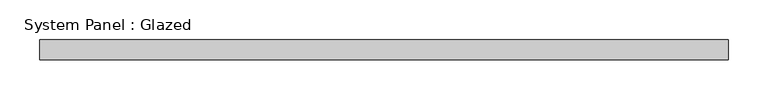
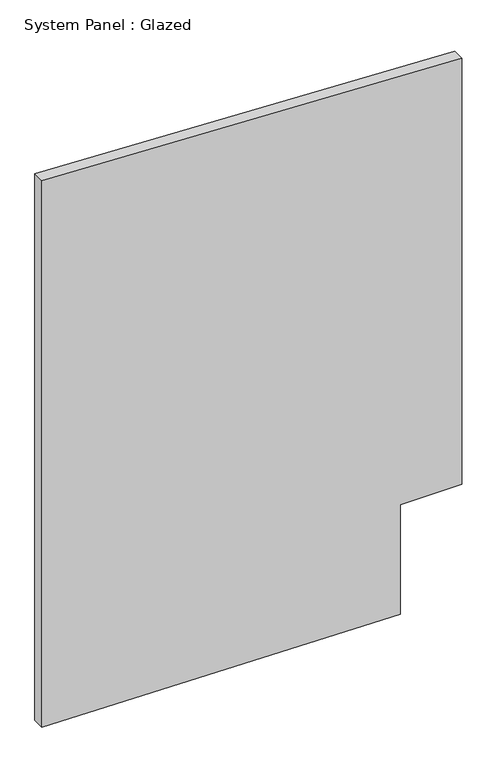
"""IFC4 building model written with IfcOpenShell, lengths in millimetres: plate geometry, System Panel : Glazed."""

import ifcopenshell
import ifcopenshell.guid

model = None  # the IFC model being written
_history = None  # IfcOwnerHistory: only IFC2X3 demands one
_inside = {}  # id of a spatial element -> (the spatial element, [elements in it])
_under = {}  # id of a project, library or spatial element -> (it, [spatial elements below it])
_declared = {}  # id of a project -> (the project, [libraries it declares])
_typed = {}  # id of a type object -> (the type object, [elements of that type])
_made_of = {}  # id of a material, layer set ... -> (it, [elements and type objects made of it])


def new_model(schema):
    """Start an empty IFC model of exactly this schema.

    Asked for "IFC4X3", IfcOpenShell would pick the latest addendum, in which some entities
    have other attributes; the version numbers below select the first issue.
    IFC2X3 requires an IfcOwnerHistory on every rooted entity: one is made here for all.
    """
    global model, _history
    if schema == "IFC4X3":
        model = ifcopenshell.file(schema_version=(4, 3, 0, 0))
    else:
        model = ifcopenshell.file(schema=schema)
    _inside.clear()
    _under.clear()
    _declared.clear()
    _typed.clear()
    _made_of.clear()
    _history = None
    if model.schema == "IFC2X3":
        org = make("IfcOrganization", Name="unknown")
        user = make(
            "IfcPersonAndOrganization",
            ThePerson=make("IfcPerson", FamilyName="unknown"),
            TheOrganization=org,
        )
        app = make(
            "IfcApplication",
            ApplicationDeveloper=org,
            Version="unknown",
            ApplicationFullName="unknown",
            ApplicationIdentifier="unknown",
        )
        _history = make(
            "IfcOwnerHistory",
            OwningUser=user,
            OwningApplication=app,
            ChangeAction="ADDED",
            CreationDate=0,
        )
    return model


def make(cls, **values):
    """One entity of the class cls with the attributes given. An attribute that is None is left unset."""
    return model.create_entity(
        cls, **{name: value for name, value in values.items() if value is not None}
    )


def rooted(cls, **values):
    """An entity with a GlobalId (a new one), such as an element, a storey or a relation."""
    return make(cls, GlobalId=ifcopenshell.guid.new(), OwnerHistory=_history, **values)


def si_unit(unit_type, name, prefix=None):
    """IfcSIUnit, for example si_unit("LENGTHUNIT", "METRE", prefix="MILLI")."""
    return make("IfcSIUnit", UnitType=unit_type, Prefix=prefix, Name=name)


def assignment(units):
    """IfcUnitAssignment: the units of a project."""
    return None if units is None else make("IfcUnitAssignment", Units=units)


def point(xyz):
    """IfcCartesianPoint."""
    return None if xyz is None else make("IfcCartesianPoint", Coordinates=xyz)


def direction(xyz):
    """IfcDirection."""
    return None if xyz is None else make("IfcDirection", DirectionRatios=xyz)


def frame(location, z_axis=None, x_axis=None):
    """IfcAxis2Placement3D, a coordinate frame: its origin and axes. An axis left out is left unset."""
    return make(
        "IfcAxis2Placement3D",
        Location=point(location),
        Axis=direction(z_axis),
        RefDirection=direction(x_axis),
    )


def origin():
    """The frame at (0, 0, 0) with its axes left unset."""
    return frame((0.0, 0.0, 0.0))


def place(relative_to, where):
    """IfcLocalPlacement: puts the frame where relative to a parent placement (None: the world)."""
    return make(
        "IfcLocalPlacement", PlacementRelTo=relative_to, RelativePlacement=where
    )


def context(
    kind, dimensions, precision=None, world=None, true_north=None, identifier=None
):
    """IfcGeometricRepresentationContext, for example the 3D "Model" context."""
    return make(
        "IfcGeometricRepresentationContext",
        ContextIdentifier=identifier,
        ContextType=kind,
        CoordinateSpaceDimension=dimensions,
        Precision=precision,
        WorldCoordinateSystem=world,
        TrueNorth=true_north,
    )


def project(units=None, contexts=None):
    """IfcProject with its units and contexts."""
    return rooted(
        "IfcProject",
        Name="project",
        RepresentationContexts=contexts,
        UnitsInContext=assignment(units),
    )


def spatial(cls, under=None, at=None, **own):
    """A site, building, storey or space (cls), placed at a placement, below another one or the project."""
    s = rooted(cls, ObjectPlacement=at, **own)
    if under is not None:
        _under.setdefault(under.id(), (under, []))[1].append(s)
    return s


def polyline(points):
    """IfcPolyline through the points."""
    return make("IfcPolyline", Points=[point(p) for p in points])


def outline(outer, holes=None, kind="AREA"):
    """IfcArbitraryClosedProfileDef: a profile drawn as a closed curve; with holes, ...WithVoids."""
    if holes is None:
        return make("IfcArbitraryClosedProfileDef", ProfileType=kind, OuterCurve=outer)
    return make(
        "IfcArbitraryProfileDefWithVoids",
        ProfileType=kind,
        OuterCurve=outer,
        InnerCurves=holes,
    )


def extrude(swept, where, along, depth):
    """IfcExtrudedAreaSolid: the profile swept, set in the frame where, extruded along a direction by depth."""
    return make(
        "IfcExtrudedAreaSolid",
        SweptArea=swept,
        Position=where,
        ExtrudedDirection=direction(along),
        Depth=depth,
    )


def shape(context_of_items, identifier, shape_type, items):
    """IfcShapeRepresentation: the items that make up one representation, for example the "Body"."""
    return make(
        "IfcShapeRepresentation",
        ContextOfItems=context_of_items,
        RepresentationIdentifier=identifier,
        RepresentationType=shape_type,
        Items=items,
    )


def source(mapping_origin, context_of_items, identifier, shape_type, items):
    """IfcRepresentationMap: a shape defined once, which mapped items show again and again."""
    return make(
        "IfcRepresentationMap",
        MappingOrigin=mapping_origin,
        MappedRepresentation=shape(context_of_items, identifier, shape_type, items),
    )


def transform(
    local_origin,
    x_axis=None,
    y_axis=None,
    z_axis=None,
    scale=None,
    scale2=None,
    scale3=None,
    uniform=True,
):
    """IfcCartesianTransformationOperator3D, or its non-uniform kind. x_axis, y_axis, z_axis: its Axis1, 2, 3."""
    if uniform:
        return make(
            "IfcCartesianTransformationOperator3D",
            Axis1=direction(x_axis),
            Axis2=direction(y_axis),
            LocalOrigin=point(local_origin),
            Scale=scale,
            Axis3=direction(z_axis),
        )
    return make(
        "IfcCartesianTransformationOperator3DnonUniform",
        Axis1=direction(x_axis),
        Axis2=direction(y_axis),
        LocalOrigin=point(local_origin),
        Scale=scale,
        Axis3=direction(z_axis),
        Scale2=scale2,
        Scale3=scale3,
    )


def mapped(mapping_source, mapping_target):
    """IfcMappedItem: shows the shape of a source again, moved by a transform."""
    return make(
        "IfcMappedItem", MappingSource=mapping_source, MappingTarget=mapping_target
    )


def made_of(thing, what):
    """Note that an element or type object is made of a material, layer set ...; save() writes the relation."""
    if what is not None:
        _made_of.setdefault(what.id(), (what, []))[1].append(thing)
    return thing


def element(
    cls,
    number,
    at=None,
    inside=None,
    cuts=None,
    type_object=None,
    material=None,
    context=None,
    identifier="Body",
    shape_type=None,
    held_by="IfcProductDefinitionShape",
    body=None,
    shapes=None,
    **own,
):
    """One element of the class cls, such as IfcWall. Its Tag is "e" and its number.

    at: its placement. inside: the storey or other place that contains it. cuts: it is an
    opening in that element (IfcRelVoidsElement). A single representation is given by context,
    identifier, shape_type and body (its items); several are given by shapes. held_by: the class
    of the entity that holds the representations. save() writes the other relations.
    """
    e = rooted(cls, Tag="e%d" % number, ObjectPlacement=at, **own)
    if body is not None:
        shapes = [shape(context, identifier, shape_type, body)]
    if shapes is not None:
        e.Representation = make(held_by, Representations=shapes)
    if inside is not None:
        _inside.setdefault(inside.id(), (inside, []))[1].append(e)
    if cuts is not None:
        rooted(
            "IfcRelVoidsElement", RelatingBuildingElement=cuts, RelatedOpeningElement=e
        )
    if type_object is not None:
        _typed.setdefault(type_object.id(), (type_object, []))[1].append(e)
    return made_of(e, material)


def aggregate(whole, parts):
    """IfcRelAggregates: a whole, such as a stair, and the parts it consists of."""
    return rooted("IfcRelAggregates", RelatingObject=whole, RelatedObjects=parts)


def save(model, path):
    """Write the relations noted so far, then the file.

    IfcRelAggregates (storeys below a building ...), IfcRelContainedInSpatialStructure (elements
    in a storey), IfcRelDefinesByType, IfcRelAssociatesMaterial and IfcRelDeclares: one each for
    every whole, place, type object, material and project.
    """
    for whole, parts in _under.values():
        aggregate(whole, parts)
    for where, things in _inside.values():
        rooted(
            "IfcRelContainedInSpatialStructure",
            RelatedElements=things,
            RelatingStructure=where,
        )
    for kind, things in _typed.values():
        rooted("IfcRelDefinesByType", RelatedObjects=things, RelatingType=kind)
    for what, things in _made_of.values():
        rooted("IfcRelAssociatesMaterial", RelatedObjects=things, RelatingMaterial=what)
    for by, libraries in _declared.values():
        rooted("IfcRelDeclares", RelatingContext=by, RelatedDefinitions=libraries)
    model.write(path)


def system_panel_glazed_6f803337(model_context):
    return source(origin(), model_context, "Body", "SweptSolid", [
        extrude(outline(polyline([(12.5542209, -434.3323712), (0.0, 307.3323712), (239.9574465, 307.3323712), (239.9574465, 434.3323712), (1172.0413931, 434.3323712), (1208.2357574, -434.3323712), (12.5542209, -434.3323712)])), frame((0.0, -12.7, 0.0), z_axis=(0.0, 1.0, 0.0), x_axis=(0.0, 0.0, 1.0)), (0.0, 0.0, 1.0), 25.4),
    ])


if __name__ == "__main__":
    model = new_model("IFC4")
    model_context = context("Model", 3, world=origin())
    ifc_project = project(units=[si_unit("LENGTHUNIT", "METRE", prefix="MILLI")], contexts=[model_context])
    site = spatial("IfcSite", under=ifc_project)
    building = spatial("IfcBuilding", under=site)
    placement = place(None, origin())
    system_panel_glazed_shape = system_panel_glazed_6f803337(model_context)
    element("IfcPlate", 1, ObjectType="System Panel : Glazed", at=placement, inside=building, context=model_context, shape_type="MappedRepresentation", body=[
        mapped(system_panel_glazed_shape, transform((0.0, 0.0, 0.0), x_axis=(1.0, 0.0, 0.0), y_axis=(0.0, 1.0, 0.0), z_axis=(0.0, 0.0, 1.0))),
    ])
    save(model, "model.ifc")

# Revit data of these elements
# Element 1 (IfcPlate, "System Panel : Glazed")
#   Materials on its faces: "BUTT GLAZED STOREFRONT WITH VERTICAL MULLION"
# Materials
#   "BUTT GLAZED STOREFRONT WITH VERTICAL MULLION": class "Glass", colour RGB 236 240 239, transparency 0.39, Description = "Soda Lime Glass", Cost = 0
